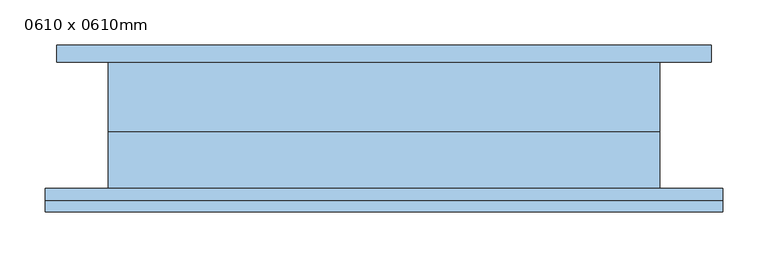
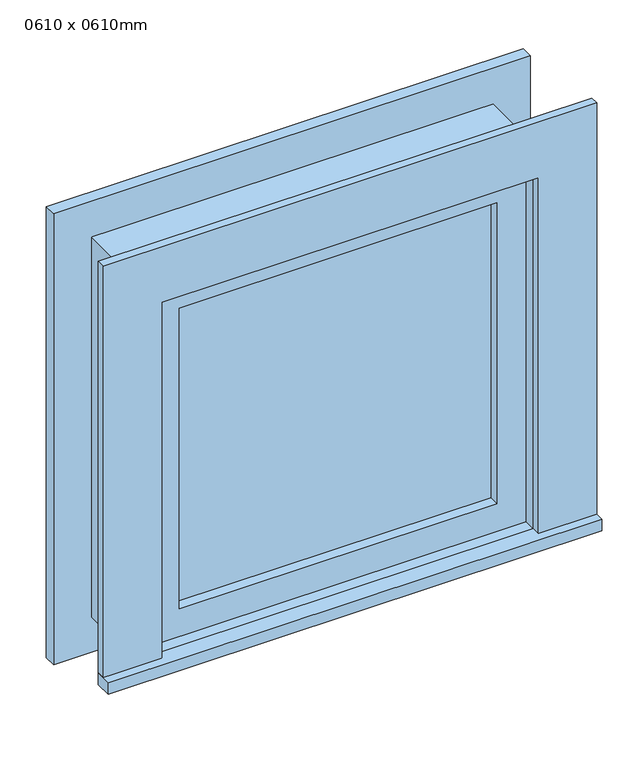
"""IFC4 building model written with IfcOpenShell, lengths in millimetres: window geometry, Travessa horizontal : 0610 x 0610mm."""

from ifc_helpers import new_model, si_unit, frame, origin, place, context, project, spatial, polyline, outline, extrude, source, transform, mapped, element, save


def window_0610_x_0610mm_29328112(model_context):
    return source(origin(), model_context, "Body", "SweptSolid", [
        extrude(outline(polyline([(-413.05, -95.7), (-413.05, -70.0), (336.85, -70.0), (336.85, -95.7), (-413.05, -95.7)])), frame((0.0, 0.0, 2159.0), z_axis=(0.0, 0.0, 1.0), x_axis=(1.0, 0.0, 0.0)), (0.0, 0.0, 1.0), 19.05),
        extrude(outline(polyline([(2749.95, -324.05), (2749.95, 247.85), (2178.05, 247.85), (2178.05, 336.85), (2838.95, 336.85), (2838.95, -413.05), (2178.05, -413.05), (2178.05, -324.05), (2749.95, -324.05)])), frame((0.0, -83.0, 0.0), z_axis=(0.0, 1.0, 0.0), x_axis=(0.0, 0.0, 1.0)), (0.0, 0.0, 1.0), 13.0),
        extrude(outline(polyline([(2826.25, 324.15), (2826.25, -400.35), (2101.75, -400.35), (2101.75, 324.15), (2826.25, 324.15)]), holes=[polyline([(2737.25, 235.15), (2190.75, 235.15), (2190.75, -311.35), (2737.25, -311.35), (2737.25, 235.15)])]), frame((0.0, 70.0, 0.0), z_axis=(0.0, 1.0, 0.0), x_axis=(0.0, 0.0, 1.0)), (0.0, 0.0, 1.0), 19.0),
        extrude(outline(polyline([(203.4, -22.425), (203.4, -35.125), (-279.6, -35.125), (-279.6, -22.425), (203.4, -22.425)])), frame((0.0, 0.0, 2222.5), z_axis=(0.0, 0.0, 1.0), x_axis=(1.0, 0.0, 0.0)), (0.0, 0.0, 1.0), 483.0),
        extrude(outline(polyline([(2749.95, -324.05), (2178.05, -324.05), (2178.05, 247.85), (2749.95, 247.85), (2749.95, -324.05)]), holes=[polyline([(2705.5, -279.6), (2705.5, 203.4), (2222.5, 203.4), (2222.5, -279.6), (2705.5, -279.6)])]), frame((0.0, -51.0, 0.0), z_axis=(0.0, 1.0, 0.0), x_axis=(0.0, 0.0, 1.0)), (0.0, 0.0, 1.0), 44.45),
        extrude(outline(polyline([(2769.0, -343.1), (2159.0, -343.1), (2159.0, 266.9), (2769.0, 266.9), (2769.0, -343.1)]), holes=[polyline([(2737.25, -311.35), (2737.25, 235.15), (2190.75, 235.15), (2190.75, -311.35), (2737.25, -311.35)])]), frame((0.0, -6.55, 0.0), z_axis=(0.0, 1.0, 0.0), x_axis=(0.0, 0.0, 1.0)), (0.0, 0.0, 1.0), 76.55),
        extrude(outline(polyline([(2769.0, 266.9), (2769.0, -343.1), (2159.0, -343.1), (2159.0, 266.9), (2769.0, 266.9)]), holes=[polyline([(2749.95, 247.85), (2178.05, 247.85), (2178.05, -324.05), (2749.95, -324.05), (2749.95, 247.85)])]), frame((0.0, -70.0, 0.0), z_axis=(0.0, 1.0, 0.0), x_axis=(0.0, 0.0, 1.0)), (0.0, 0.0, 1.0), 63.45),
    ])


if __name__ == "__main__":
    model = new_model("IFC4")
    model_context = context("Model", 3, world=origin())
    ifc_project = project(units=[si_unit("LENGTHUNIT", "METRE", prefix="MILLI")], contexts=[model_context])
    site = spatial("IfcSite", under=ifc_project)
    building = spatial("IfcBuilding", under=site)
    placement = place(None, origin())
    window_0610_x_0610mm_shape = window_0610_x_0610mm_29328112(model_context)
    element("IfcWindow", 1, ObjectType="Travessa horizontal : 0610 x 0610mm", at=placement, inside=building, context=model_context, shape_type="MappedRepresentation", body=[
        mapped(window_0610_x_0610mm_shape, transform((0.0, 0.0, 0.0), x_axis=(1.0, 0.0, 0.0), y_axis=(0.0, 1.0, 0.0), z_axis=(0.0, 0.0, 1.0))),
    ])
    save(model, "model.ifc")

# Revit data of these elements
# Type "Travessa horizontal : 0610 x 0610mm"
#   Type Mark = "EF31"
#   Construction Type Id = "GSP4R"
#   Analytic Construction = "Vidraça única Pilkington 1/8 pol"
#   Visual Light Transmittance = 0.9
#   Solar Heat Gain Coefficient = 0.78
#   Heat Transfer Coefficient (U) = 3.6886 W/(m²·K)
#   Height = 0.610 m
#   Altura-padrão do peitoril = 2.159 m
#   Projeção da apara - Ext. = 0.013 m
#   Projeção da apara - Int. = 0.019 m
#   Largura da apara - Exterior = 0.089 m
#   Largura da apara - Interior = 0.089 m
#   Width = 0.610 m
#   Janela aplicada = 0.019 m
#   Define Thermal Properties by = 1
#   Material do painel de vidro = Vidro
#   Material do caixilho = Caixilho
#   Material da apara externa = Recortar
#   Material da apara interna = Recortar
#   Wall Closure = (empty or 0)
# Element 1 (IfcWindow, "Travessa horizontal : 0610 x 0610mm")
#   Materials on its faces: "Recortar", "Caixilho", "Vidro"
# Materials
#   "Vidro": class "Vidro", colour RGB 0 128 192, transparency 0.9, Description = "Vidro de sílica", Cost = 0
#   "Caixilho": class "Madeira", colour RGB 224 178 126, transparency 0
#   "Recortar": class "Madeira", colour RGB 224 178 126, transparency 0
